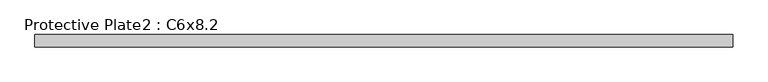
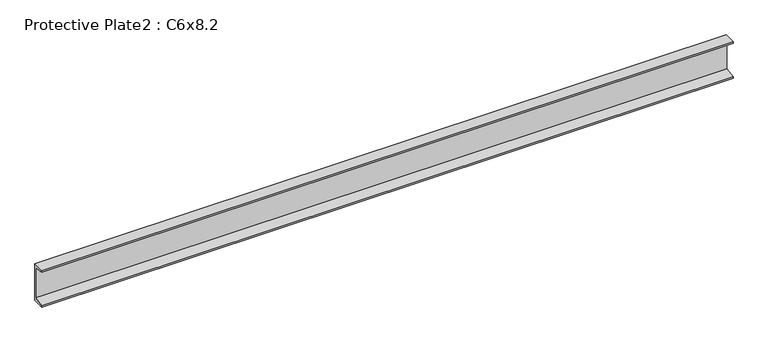
"""IFC4 building model written with IfcOpenShell, lengths in millimetres: proxy geometry, Protective Plate2 : C6x8.2."""

from ifc_helpers import new_model, si_unit, frame, origin, place, context, project, spatial, polyline, outline, extrude, source, transform, mapped, element, save


def protective_plate2_c6x8_2_0d7b6ffb(model_context):
    return source(origin(), model_context, "Body", "SweptSolid", [
        extrude(outline(polyline([(-536340.3753841, 914.4), (-536291.6073841, 914.4), (-536291.6073841, 762.0), (-536340.3753841, 762.0), (-536340.3753841, 767.08), (-536296.6675403, 774.7868721), (-536296.6675403, 901.6131279), (-536340.3753841, 909.32), (-536340.3753841, 914.4)])), frame((587467.4934739, 0.0, 0.0), z_axis=(1.0, 0.0, 0.0), x_axis=(0.0, 1.0, 0.0)), (0.0, 0.0, 1.0), 2749.55),
    ])


if __name__ == "__main__":
    model = new_model("IFC4")
    model_context = context("Model", 3, world=origin())
    ifc_project = project(units=[si_unit("LENGTHUNIT", "METRE", prefix="MILLI")], contexts=[model_context])
    site = spatial("IfcSite", under=ifc_project)
    building = spatial("IfcBuilding", under=site)
    placement = place(None, origin())
    protective_plate2_c6x8_2_shape = protective_plate2_c6x8_2_0d7b6ffb(model_context)
    element("IfcBuildingElementProxy", 1, Name="Protective Plate2 : C6x8.2", ObjectType="Protective Plate2 : C6x8.2", at=placement, inside=building, context=model_context, shape_type="MappedRepresentation", body=[
        mapped(protective_plate2_c6x8_2_shape, transform((0.0, 0.0, 0.0), x_axis=(1.0, 0.0, 0.0), y_axis=(0.0, 1.0, 0.0), z_axis=(0.0, 0.0, 1.0))),
    ])
    save(model, "model.ifc")

# Revit data of these elements
# Element 1 (IfcBuildingElementProxy, "Protective Plate2 : C6x8.2")
#   Materials on its faces: "C6x8.2 GALV CHANNEL"
# Materials
#   "C6x8.2 GALV CHANNEL": class "Generic", colour RGB 211 211 207, transparency 0, Cost = 0
